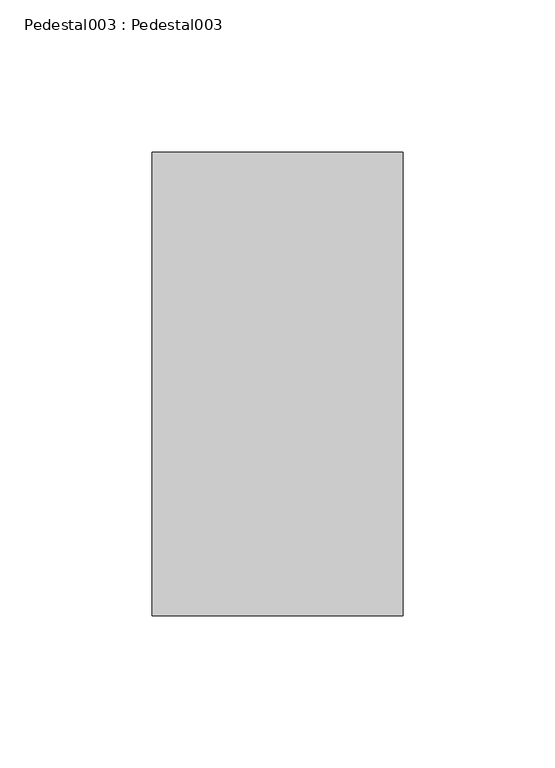
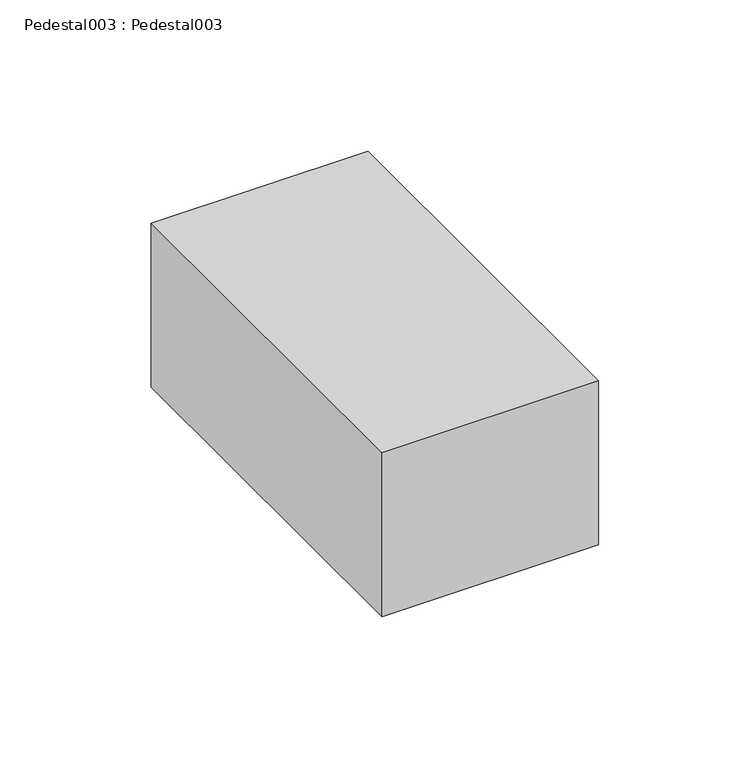
"""IFC4 building model written with IfcOpenShell, lengths in millimetres: proxy geometry, Pedestal003 : Pedestal003."""

from ifc_helpers import new_model, si_unit, frame, origin, place, context, project, spatial, polyline, outline, extrude, source, transform, mapped, element, save


def pedestal003_pedestal003_a9b3681d(model_context):
    return source(origin(), model_context, "Body", "SweptSolid", [
        extrude(outline(polyline([(-6478.9810059, 9829.7531721), (-6561.5310059, 9829.7531721), (-6561.5310059, 9982.1531721), (-6478.9810059, 9982.1531721), (-6478.9810059, 9829.7531721)])), frame((0.0, 0.0, 40115.171875), z_axis=(0.0, 0.0, 1.0), x_axis=(1.0, 0.0, 0.0)), (0.0, 0.0, 1.0), 66.061023),
    ])


if __name__ == "__main__":
    model = new_model("IFC4")
    model_context = context("Model", 3, world=origin())
    ifc_project = project(units=[si_unit("LENGTHUNIT", "METRE", prefix="MILLI")], contexts=[model_context])
    site = spatial("IfcSite", under=ifc_project)
    building = spatial("IfcBuilding", under=site)
    placement = place(None, origin())
    pedestal003_pedestal003_shape = pedestal003_pedestal003_a9b3681d(model_context)
    element("IfcBuildingElementProxy", 1, Name="Pedestal003 : Pedestal003", ObjectType="Pedestal003 : Pedestal003", at=placement, inside=building, context=model_context, shape_type="MappedRepresentation", body=[
        mapped(pedestal003_pedestal003_shape, transform((0.0, 0.0, 0.0), x_axis=(1.0, 0.0, 0.0), y_axis=(0.0, 1.0, 0.0), z_axis=(0.0, 0.0, 1.0))),
    ])
    save(model, "model.ifc")

# Revit data of these elements
# Type "Pedestal003 : Pedestal003"
#   NameOverride = "Pedestal003"
# Element 1 (IfcBuildingElementProxy, "Pedestal003 : Pedestal003")
#   Materials on its faces: "BUZON PEDESTAL"
# Materials
#   "BUZON PEDESTAL": class "Unassigned", colour RGB 66 66 66, transparency 0
